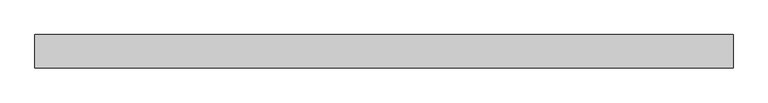
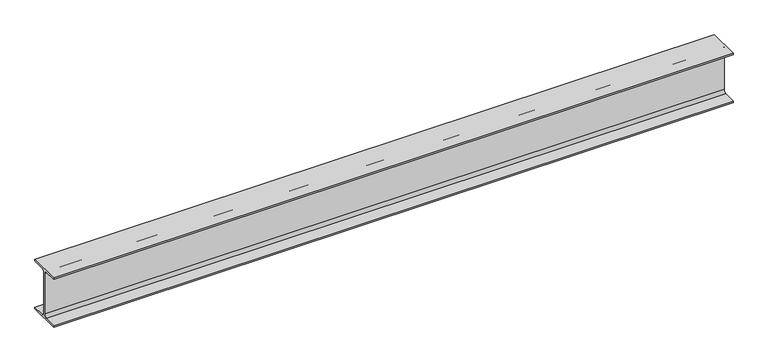
"""IFC4 building model written with IfcOpenShell, lengths in millimetres: beam geometry, 0912_Steel Framing_H-KSD3502 : H_SB_ASB_H-482x300x11x15."""

from ifc_helpers import new_model, si_unit, point, frame, frame_2d, origin, place, context, project, spatial, polyline, circle_curve, trimmed, segment, composite_curve, outline, extrude, source, transform, mapped, element, save


def beam_79f0d603(model_context):
    return source(origin(), model_context, "Body", "SweptSolid", [
        extrude(outline(composite_curve([segment(polyline([(150.0, -226.0), (150.0, -241.0), (-150.0, -241.0), (-150.0, -226.0), (-31.5, -226.0)]), True, "CONTINUOUS"), segment(trimmed(circle_curve(frame_2d((-31.5, -200.0)), 26.0), [point((-31.5, -226.0))], [point((-5.5, -200.0))], True, "CARTESIAN"), True, "CONTINUOUS"), segment(polyline([(-5.5, -200.0), (-5.5, 200.0)]), True, "CONTINUOUS"), segment(trimmed(circle_curve(frame_2d((-31.5, 200.0)), 26.0), [point((-5.5, 200.0))], [point((-31.5, 226.0))], True, "CARTESIAN"), True, "CONTINUOUS"), segment(polyline([(-31.5, 226.0), (-150.0, 226.0), (-150.0, 241.0), (150.0, 241.0), (150.0, 226.0), (31.5, 226.0)]), True, "CONTINUOUS"), segment(trimmed(circle_curve(frame_2d((31.5, 200.0)), 26.0), [point((31.5, 226.0))], [point((5.5, 200.0))], True, "CARTESIAN"), True, "CONTINUOUS"), segment(polyline([(5.5, 200.0), (5.5, -200.0)]), True, "CONTINUOUS"), segment(trimmed(circle_curve(frame_2d((31.5, -200.0)), 26.0), [point((5.5, -200.0))], [point((31.5, -226.0))], True, "CARTESIAN"), True, "CONTINUOUS"), segment(polyline([(31.5, -226.0), (150.0, -226.0)]), True, "CONTINUOUS")], self_intersect=False)), frame((-3154.8, 0.0, 0.0), z_axis=(1.0, 0.0, 0.0), x_axis=(0.0, 1.0, 0.0)), (0.0, 0.0, 1.0), 6309.6),
    ])


if __name__ == "__main__":
    model = new_model("IFC4")
    model_context = context("Model", 3, world=origin())
    ifc_project = project(units=[si_unit("LENGTHUNIT", "METRE", prefix="MILLI")], contexts=[model_context])
    site = spatial("IfcSite", under=ifc_project)
    building = spatial("IfcBuilding", under=site)
    placement = place(None, origin())
    beam_shape = beam_79f0d603(model_context)
    element("IfcBeam", 1, ObjectType="0912_Steel Framing_H-KSD3502 : H_SB_ASB_H-482x300x11x15", at=placement, inside=building, context=model_context, shape_type="MappedRepresentation", body=[
        mapped(beam_shape, transform((0.0, 0.0, 0.0), x_axis=(1.0, 0.0, 0.0), y_axis=(0.0, 1.0, 0.0), z_axis=(0.0, 0.0, 1.0))),
    ])
    save(model, "model.ifc")

# Revit data of these elements
# Type "0912_Steel Framing_H-KSD3502 : H_SB_ASB_H-482x300x11x15"
#   H_WM Code_1 = "S01AA001-00001 | Main Steel Structure Fabrication Work | Shelter/Building | Heavy Steel - Standard (Weight≥90KG/M) | Material: (   )"
#   H_WM Code_2 = "S03AA027-00001 | Main Steel Structure Erection Work | Shelter/Building | Heavy Steel (Weight≥90KG/M) | Material: (   )"
#   H_WM Code_3 = "S01AA010-00001 | Main Steel Structure Fabrication Work | Shelter/Building | Steel Painting/Coating | for Non-Fireproofed Steel Surface, Surface Preparation, Primer, Second & Final Coat | Material: (   )"
#   H_Q'ty Cal Type Tag = "SB-Q2"
#   Width = 30.0 cm
#   Web Thickness = 1.1 cm
#   Web Fillet = 2.6 cm
#   Warping Constant = 3680000.0 cm⁶
#   W = 0
#   Torsional Moment of Inertia = 88.2192 cm⁴
#   Section Area = 145.5 cm²
#   Plastic Modulus weak axis = 695.0 cm³
#   Plastic Modulus strong axis = 2790.0 cm³
#   Perimeter = 2.10 m²/m
#   Nominal Weight = 114.00 kgf/m
#   Moment of Inertia weak axis = 6760.00 cm⁴
#   Moment of Inertia strong axis = 60400.00 cm⁴
#   Height = 48.2 cm
#   Flange Thickness = 1.5 cm
#   Elastic Modulus weak axis = 451.0 cm³
#   Elastic Modulus strong axis = 2500.0 cm³
#   Centroid Vertical = 24.1 cm
#   Centroid Horizontal = 15.0 cm
#   Ix = 604000000
#   Length [instance default] = 1.5240 m
#   Zx = 2790000
#   b = 0.3000 m
#   h = 0.4820 m
#   r = 0.0260 m
#   s = 0.0110 m
#   t = 0.0150 m
#   A = 0.01455 m²
#   Structural Material [instance default] = Steel, 45-345
#   Assembly Code = ""
# Element 1 (IfcBeam, "0912_Steel Framing_H-KSD3502 : H_SB_ASB_H-482x300x11x15")
#   Structural Material = none
# Materials
#   "Steel, 45-345": class "Metal", colour RGB 189 187 185, transparency 0, Description = "Steel 345 MPa", Cost = 0
